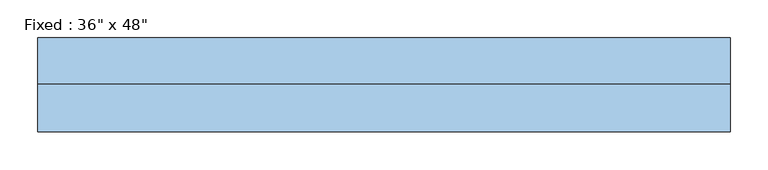
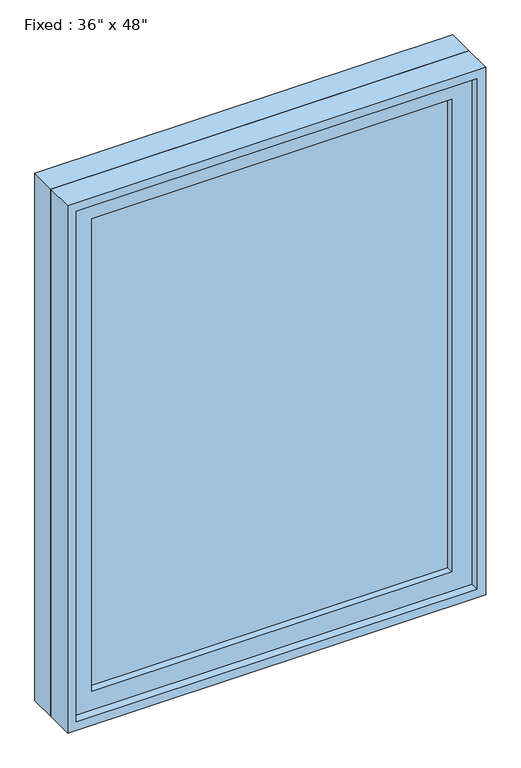
"""IFC4 building model written with IfcOpenShell, lengths in millimetres: window geometry."""

from ifc_helpers import new_model, si_unit, frame, origin, place, context, project, spatial, polyline, outline, extrude, source, transform, mapped, element, save


def window_254735d6(model_context):
    return source(origin(), model_context, "Body", "SweptSolid", [
        extrude(outline(polyline([(355.6, -14.2875), (355.6, -26.9875), (-431.8, -26.9875), (-431.8, -14.2875), (355.6, -14.2875)])), frame((0.0, 0.0, 977.9), z_axis=(0.0, 0.0, 1.0), x_axis=(1.0, 0.0, 0.0)), (0.0, 0.0, 1.0), 1092.2),
        extrude(outline(polyline([(2114.55, -476.25), (933.45, -476.25), (933.45, 400.05), (2114.55, 400.05), (2114.55, -476.25)]), holes=[polyline([(2070.1, -431.8), (2070.1, 355.6), (977.9, 355.6), (977.9, -431.8), (2070.1, -431.8)])]), frame((0.0, -42.8625, 0.0), z_axis=(0.0, 1.0, 0.0), x_axis=(0.0, 0.0, 1.0)), (0.0, 0.0, 1.0), 44.45),
        extrude(outline(polyline([(2133.6, -495.3), (914.4, -495.3), (914.4, 419.1), (2133.6, 419.1), (2133.6, -495.3)]), holes=[polyline([(2101.85, -463.55), (2101.85, 387.35), (946.15, 387.35), (946.15, -463.55), (2101.85, -463.55)])]), frame((0.0, 1.5875, 0.0), z_axis=(0.0, 1.0, 0.0), x_axis=(0.0, 0.0, 1.0)), (0.0, 0.0, 1.0), 60.325),
        extrude(outline(polyline([(2133.6, 419.1), (2133.6, -495.3), (914.4, -495.3), (914.4, 419.1), (2133.6, 419.1)]), holes=[polyline([(2114.55, 400.05), (933.45, 400.05), (933.45, -476.25), (2114.55, -476.25), (2114.55, 400.05)])]), frame((0.0, -61.9125, 0.0), z_axis=(0.0, 1.0, 0.0), x_axis=(0.0, 0.0, 1.0)), (0.0, 0.0, 1.0), 63.5),
    ])


if __name__ == "__main__":
    model = new_model("IFC4")
    model_context = context("Model", 3, world=origin())
    ifc_project = project(units=[si_unit("LENGTHUNIT", "METRE", prefix="MILLI")], contexts=[model_context])
    site = spatial("IfcSite", under=ifc_project)
    building = spatial("IfcBuilding", under=site)
    placement = place(None, origin())
    window_shape = window_254735d6(model_context)
    element("IfcWindow", 1, ObjectType="Fixed : 36\" x 48\"", at=placement, inside=building, context=model_context, shape_type="MappedRepresentation", body=[
        mapped(window_shape, transform((0.0, 0.0, 0.0), x_axis=(1.0, 0.0, 0.0), y_axis=(0.0, 1.0, 0.0), z_axis=(0.0, 0.0, 1.0))),
    ])
    save(model, "model.ifc")

# Revit data of these elements
# Type "Fixed : 36\" x 48\""
#   Type Mark = "1"
#   Assembly Code = "B2020100"
#   Height = 4' - 0"
#   Default Sill Height = 3' - 0"
#   Width = 3' - 0"
#   Window Inset = 0' - 0 3/4"
#   Glass Pane Material = Glass
#   Sash Material = Sash
#   Wall Closure = (empty or 0)
# Element 1 (IfcWindow, "Fixed : 36\" x 48\"")
#   Materials on its faces: "Sash", "Glass"
# Materials
#   "Glass": class "Glass", colour RGB 0 128 192, transparency 0.75
#   "Sash": class "Wood", colour RGB 224 178 126, transparency 0
